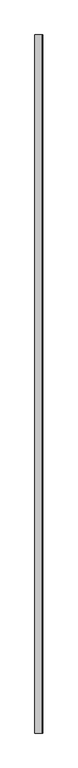
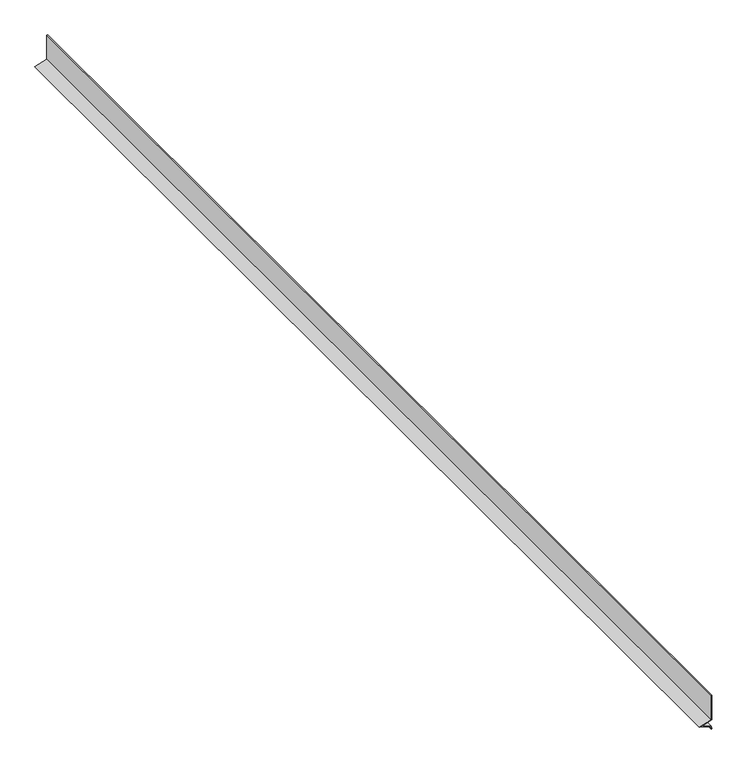
"""IFC4 building model written with IfcOpenShell, lengths in millimetres: proxy geometry, Metal profile025 233 : Metal profile025 233."""

from ifc_helpers import new_model, si_unit, frame, origin, place, context, project, spatial, polyline, outline, extrude, source, transform, mapped, element, save


def generic_models_e0bbe71d(model_context):
    return source(origin(), model_context, "Body", "SweptSolid", [
        extrude(outline(polyline([(33322.0337932, -9678.6315139), (33327.1485436, -9679.594709), (33332.6487015, -9696.7063117), (33338.458458, -9678.6315139), (33383.4487015, -9678.6315139), (33383.4487015, -9679.9015139), (33339.3842373, -9679.9015139), (33332.6487015, -9700.8565139), (33326.1707534, -9680.7028974), (33321.7987616, -9679.8795765), (33322.0337932, -9678.6315139)])), frame((0.0, 7982.1529359, 0.0), z_axis=(0.0, 1.0, 0.0), x_axis=(0.0, 0.0, 1.0)), (0.0, 0.0, 1.0), 2000.0),
    ])


if __name__ == "__main__":
    model = new_model("IFC4")
    model_context = context("Model", 3, world=origin())
    ifc_project = project(units=[si_unit("LENGTHUNIT", "METRE", prefix="MILLI")], contexts=[model_context])
    site = spatial("IfcSite", under=ifc_project)
    building = spatial("IfcBuilding", under=site)
    placement = place(None, origin())
    generic_models_shape = generic_models_e0bbe71d(model_context)
    element("IfcBuildingElementProxy", 1, Name="Metal profile025 233 : Metal profile025 233", ObjectType="Metal profile025 233 : Metal profile025 233", at=placement, inside=building, context=model_context, shape_type="MappedRepresentation", body=[
        mapped(generic_models_shape, transform((0.0, 0.0, 0.0), x_axis=(1.0, 0.0, 0.0), y_axis=(0.0, 1.0, 0.0), z_axis=(0.0, 0.0, 1.0))),
    ])
    save(model, "model.ifc")

# Revit data of these elements
# Type "Metal profile025 233 : Metal profile025 233"
#   NameOverride = "Metal profile025"
# Element 1 (IfcBuildingElementProxy, "Metal profile025 233 : Metal profile025 233")
#   Materials on its faces: "16 GA. COPPER WEEP SCREED W/ MIN 3 1/2\" ATTACHMENT FLANGE - LAP UNDERLAYMENT OVER WEED SCREED"
# Materials
#   "16 GA. COPPER WEEP SCREED W/ MIN 3 1/2\" ATTACHMENT FLANGE - LAP UNDERLAYMENT OVER WEED SCREED": class "Unassigned", colour RGB 251 232 155, transparency 0, Cost = 0
